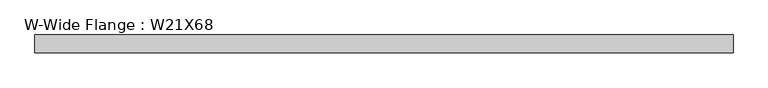
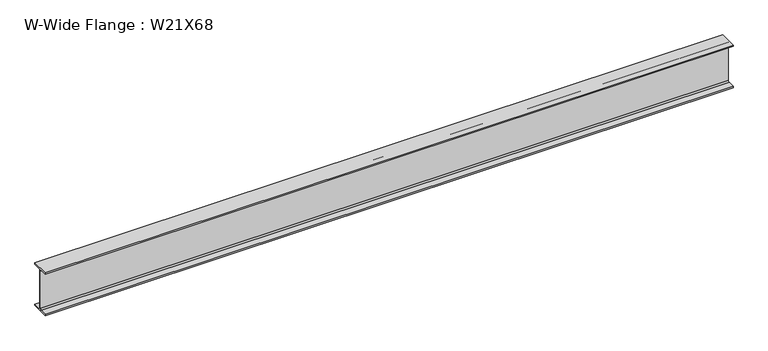
"""IFC4 building model written with IfcOpenShell, lengths in millimetres: beam geometry, W-Wide Flange : W21X68."""

import ifcopenshell
import ifcopenshell.guid

model = None  # the IFC model being written
_history = None  # IfcOwnerHistory: only IFC2X3 demands one
_inside = {}  # id of a spatial element -> (the spatial element, [elements in it])
_under = {}  # id of a project, library or spatial element -> (it, [spatial elements below it])
_declared = {}  # id of a project -> (the project, [libraries it declares])
_typed = {}  # id of a type object -> (the type object, [elements of that type])
_made_of = {}  # id of a material, layer set ... -> (it, [elements and type objects made of it])


def new_model(schema):
    """Start an empty IFC model of exactly this schema.

    Asked for "IFC4X3", IfcOpenShell would pick the latest addendum, in which some entities
    have other attributes; the version numbers below select the first issue.
    IFC2X3 requires an IfcOwnerHistory on every rooted entity: one is made here for all.
    """
    global model, _history
    if schema == "IFC4X3":
        model = ifcopenshell.file(schema_version=(4, 3, 0, 0))
    else:
        model = ifcopenshell.file(schema=schema)
    _inside.clear()
    _under.clear()
    _declared.clear()
    _typed.clear()
    _made_of.clear()
    _history = None
    if model.schema == "IFC2X3":
        org = make("IfcOrganization", Name="unknown")
        user = make(
            "IfcPersonAndOrganization",
            ThePerson=make("IfcPerson", FamilyName="unknown"),
            TheOrganization=org,
        )
        app = make(
            "IfcApplication",
            ApplicationDeveloper=org,
            Version="unknown",
            ApplicationFullName="unknown",
            ApplicationIdentifier="unknown",
        )
        _history = make(
            "IfcOwnerHistory",
            OwningUser=user,
            OwningApplication=app,
            ChangeAction="ADDED",
            CreationDate=0,
        )
    return model


def make(cls, **values):
    """One entity of the class cls with the attributes given. An attribute that is None is left unset."""
    return model.create_entity(
        cls, **{name: value for name, value in values.items() if value is not None}
    )


def rooted(cls, **values):
    """An entity with a GlobalId (a new one), such as an element, a storey or a relation."""
    return make(cls, GlobalId=ifcopenshell.guid.new(), OwnerHistory=_history, **values)


def si_unit(unit_type, name, prefix=None):
    """IfcSIUnit, for example si_unit("LENGTHUNIT", "METRE", prefix="MILLI")."""
    return make("IfcSIUnit", UnitType=unit_type, Prefix=prefix, Name=name)


def assignment(units):
    """IfcUnitAssignment: the units of a project."""
    return None if units is None else make("IfcUnitAssignment", Units=units)


def point(xyz):
    """IfcCartesianPoint."""
    return None if xyz is None else make("IfcCartesianPoint", Coordinates=xyz)


def direction(xyz):
    """IfcDirection."""
    return None if xyz is None else make("IfcDirection", DirectionRatios=xyz)


def frame(location, z_axis=None, x_axis=None):
    """IfcAxis2Placement3D, a coordinate frame: its origin and axes. An axis left out is left unset."""
    return make(
        "IfcAxis2Placement3D",
        Location=point(location),
        Axis=direction(z_axis),
        RefDirection=direction(x_axis),
    )


def frame_2d(location, x_axis=None):
    """IfcAxis2Placement2D, a coordinate frame in the plane: its origin and x axis."""
    return make(
        "IfcAxis2Placement2D", Location=point(location), RefDirection=direction(x_axis)
    )


def origin():
    """The frame at (0, 0, 0) with its axes left unset."""
    return frame((0.0, 0.0, 0.0))


def place(relative_to, where):
    """IfcLocalPlacement: puts the frame where relative to a parent placement (None: the world)."""
    return make(
        "IfcLocalPlacement", PlacementRelTo=relative_to, RelativePlacement=where
    )


def context(
    kind, dimensions, precision=None, world=None, true_north=None, identifier=None
):
    """IfcGeometricRepresentationContext, for example the 3D "Model" context."""
    return make(
        "IfcGeometricRepresentationContext",
        ContextIdentifier=identifier,
        ContextType=kind,
        CoordinateSpaceDimension=dimensions,
        Precision=precision,
        WorldCoordinateSystem=world,
        TrueNorth=true_north,
    )


def project(units=None, contexts=None):
    """IfcProject with its units and contexts."""
    return rooted(
        "IfcProject",
        Name="project",
        RepresentationContexts=contexts,
        UnitsInContext=assignment(units),
    )


def spatial(cls, under=None, at=None, **own):
    """A site, building, storey or space (cls), placed at a placement, below another one or the project."""
    s = rooted(cls, ObjectPlacement=at, **own)
    if under is not None:
        _under.setdefault(under.id(), (under, []))[1].append(s)
    return s


def polyline(points):
    """IfcPolyline through the points."""
    return make("IfcPolyline", Points=[point(p) for p in points])


def circle_curve(where, radius):
    """IfcCircle in the frame where."""
    return make("IfcCircle", Position=where, Radius=radius)


def trimmed(basis, trim1, trim2, sense, master):
    """IfcTrimmedCurve: the piece of a basis curve between two trims."""
    return make(
        "IfcTrimmedCurve",
        BasisCurve=basis,
        Trim1=trim1,
        Trim2=trim2,
        SenseAgreement=sense,
        MasterRepresentation=master,
    )


def segment(curve, same_sense, transition):
    """IfcCompositeCurveSegment."""
    return make(
        "IfcCompositeCurveSegment",
        Transition=transition,
        SameSense=same_sense,
        ParentCurve=curve,
    )


def composite_curve(segments, self_intersect=None):
    """IfcCompositeCurve: segments joined end to end."""
    return make("IfcCompositeCurve", Segments=segments, SelfIntersect=self_intersect)


def outline(outer, holes=None, kind="AREA"):
    """IfcArbitraryClosedProfileDef: a profile drawn as a closed curve; with holes, ...WithVoids."""
    if holes is None:
        return make("IfcArbitraryClosedProfileDef", ProfileType=kind, OuterCurve=outer)
    return make(
        "IfcArbitraryProfileDefWithVoids",
        ProfileType=kind,
        OuterCurve=outer,
        InnerCurves=holes,
    )


def extrude(swept, where, along, depth):
    """IfcExtrudedAreaSolid: the profile swept, set in the frame where, extruded along a direction by depth."""
    return make(
        "IfcExtrudedAreaSolid",
        SweptArea=swept,
        Position=where,
        ExtrudedDirection=direction(along),
        Depth=depth,
    )


def shape(context_of_items, identifier, shape_type, items):
    """IfcShapeRepresentation: the items that make up one representation, for example the "Body"."""
    return make(
        "IfcShapeRepresentation",
        ContextOfItems=context_of_items,
        RepresentationIdentifier=identifier,
        RepresentationType=shape_type,
        Items=items,
    )


def source(mapping_origin, context_of_items, identifier, shape_type, items):
    """IfcRepresentationMap: a shape defined once, which mapped items show again and again."""
    return make(
        "IfcRepresentationMap",
        MappingOrigin=mapping_origin,
        MappedRepresentation=shape(context_of_items, identifier, shape_type, items),
    )


def transform(
    local_origin,
    x_axis=None,
    y_axis=None,
    z_axis=None,
    scale=None,
    scale2=None,
    scale3=None,
    uniform=True,
):
    """IfcCartesianTransformationOperator3D, or its non-uniform kind. x_axis, y_axis, z_axis: its Axis1, 2, 3."""
    if uniform:
        return make(
            "IfcCartesianTransformationOperator3D",
            Axis1=direction(x_axis),
            Axis2=direction(y_axis),
            LocalOrigin=point(local_origin),
            Scale=scale,
            Axis3=direction(z_axis),
        )
    return make(
        "IfcCartesianTransformationOperator3DnonUniform",
        Axis1=direction(x_axis),
        Axis2=direction(y_axis),
        LocalOrigin=point(local_origin),
        Scale=scale,
        Axis3=direction(z_axis),
        Scale2=scale2,
        Scale3=scale3,
    )


def mapped(mapping_source, mapping_target):
    """IfcMappedItem: shows the shape of a source again, moved by a transform."""
    return make(
        "IfcMappedItem", MappingSource=mapping_source, MappingTarget=mapping_target
    )


def made_of(thing, what):
    """Note that an element or type object is made of a material, layer set ...; save() writes the relation."""
    if what is not None:
        _made_of.setdefault(what.id(), (what, []))[1].append(thing)
    return thing


def element(
    cls,
    number,
    at=None,
    inside=None,
    cuts=None,
    type_object=None,
    material=None,
    context=None,
    identifier="Body",
    shape_type=None,
    held_by="IfcProductDefinitionShape",
    body=None,
    shapes=None,
    **own,
):
    """One element of the class cls, such as IfcWall. Its Tag is "e" and its number.

    at: its placement. inside: the storey or other place that contains it. cuts: it is an
    opening in that element (IfcRelVoidsElement). A single representation is given by context,
    identifier, shape_type and body (its items); several are given by shapes. held_by: the class
    of the entity that holds the representations. save() writes the other relations.
    """
    e = rooted(cls, Tag="e%d" % number, ObjectPlacement=at, **own)
    if body is not None:
        shapes = [shape(context, identifier, shape_type, body)]
    if shapes is not None:
        e.Representation = make(held_by, Representations=shapes)
    if inside is not None:
        _inside.setdefault(inside.id(), (inside, []))[1].append(e)
    if cuts is not None:
        rooted(
            "IfcRelVoidsElement", RelatingBuildingElement=cuts, RelatedOpeningElement=e
        )
    if type_object is not None:
        _typed.setdefault(type_object.id(), (type_object, []))[1].append(e)
    return made_of(e, material)


def aggregate(whole, parts):
    """IfcRelAggregates: a whole, such as a stair, and the parts it consists of."""
    return rooted("IfcRelAggregates", RelatingObject=whole, RelatedObjects=parts)


def save(model, path):
    """Write the relations noted so far, then the file.

    IfcRelAggregates (storeys below a building ...), IfcRelContainedInSpatialStructure (elements
    in a storey), IfcRelDefinesByType, IfcRelAssociatesMaterial and IfcRelDeclares: one each for
    every whole, place, type object, material and project.
    """
    for whole, parts in _under.values():
        aggregate(whole, parts)
    for where, things in _inside.values():
        rooted(
            "IfcRelContainedInSpatialStructure",
            RelatedElements=things,
            RelatingStructure=where,
        )
    for kind, things in _typed.values():
        rooted("IfcRelDefinesByType", RelatedObjects=things, RelatingType=kind)
    for what, things in _made_of.values():
        rooted("IfcRelAssociatesMaterial", RelatedObjects=things, RelatingMaterial=what)
    for by, libraries in _declared.values():
        rooted("IfcRelDeclares", RelatingContext=by, RelatedDefinitions=libraries)
    model.write(path)


def w_wide_flange_w21x68_eecb351a(model_context):
    return source(origin(), model_context, "Body", "SweptSolid", [
        extrude(outline(composite_curve([segment(polyline([(105.029, -250.571), (105.029, -267.97), (-105.029, -267.97), (-105.029, -250.571), (-22.987, -250.571)]), True, "CONTINUOUS"), segment(trimmed(circle_curve(frame_2d((-22.987, -233.045)), 17.526), [point((-22.987, -250.571))], [point((-5.461, -233.045))], True, "CARTESIAN"), True, "CONTINUOUS"), segment(polyline([(-5.461, -233.045), (-5.461, 233.045)]), True, "CONTINUOUS"), segment(trimmed(circle_curve(frame_2d((-22.987, 233.045)), 17.526), [point((-5.461, 233.045))], [point((-22.987, 250.571))], True, "CARTESIAN"), True, "CONTINUOUS"), segment(polyline([(-22.987, 250.571), (-105.029, 250.571), (-105.029, 267.97), (105.029, 267.97), (105.029, 250.571), (22.987, 250.571)]), True, "CONTINUOUS"), segment(trimmed(circle_curve(frame_2d((22.987, 233.045)), 17.526), [point((22.987, 250.571))], [point((5.461, 233.045))], True, "CARTESIAN"), True, "CONTINUOUS"), segment(polyline([(5.461, 233.045), (5.461, -233.045)]), True, "CONTINUOUS"), segment(trimmed(circle_curve(frame_2d((22.987, -233.045)), 17.526), [point((5.461, -233.045))], [point((22.987, -250.571))], True, "CARTESIAN"), True, "CONTINUOUS"), segment(polyline([(22.987, -250.571), (105.029, -250.571)]), True, "CONTINUOUS")], self_intersect=False)), frame((-4076.7, 0.0, 0.0), z_axis=(1.0, 0.0, 0.0), x_axis=(0.0, 1.0, 0.0)), (0.0, 0.0, 1.0), 8153.4),
    ])


if __name__ == "__main__":
    model = new_model("IFC4")
    model_context = context("Model", 3, world=origin())
    ifc_project = project(units=[si_unit("LENGTHUNIT", "METRE", prefix="MILLI")], contexts=[model_context])
    site = spatial("IfcSite", under=ifc_project)
    building = spatial("IfcBuilding", under=site)
    placement = place(None, origin())
    w_wide_flange_w21x68_shape = w_wide_flange_w21x68_eecb351a(model_context)
    element("IfcBeam", 1, ObjectType="W-Wide Flange : W21X68", at=placement, inside=building, context=model_context, shape_type="MappedRepresentation", body=[
        mapped(w_wide_flange_w21x68_shape, transform((0.0, 0.0, 0.0), x_axis=(1.0, 0.0, 0.0), y_axis=(0.0, 1.0, 0.0), z_axis=(0.0, 0.0, 1.0))),
    ])
    save(model, "model.ifc")

# Revit data of these elements
# Type "W-Wide Flange : W21X68"
#   Assembly Code = "B10"
#   W = 68
#   Length [instance default] = 5' - 0"
#   bf = 0' - 8.27"
#   d = 1' - 9.1"
#   k = 0' - 1 3/8"
#   k2 = 0' - 0.69"
#   tf = 0' - 0.685"
#   tw = 0' - 0.43"
#   A = 0.138889 SF
#   Structural Material [instance default] = Steel ASTM A992
# Element 1 (IfcBeam, "W-Wide Flange : W21X68")
#   Materials on its faces: "Steel ASTM A992"
# Materials
#   "Steel ASTM A992": class "Metal", colour RGB 199 199 199, transparency 0, Description = "Structural steel 50ksi", Cost = 0
